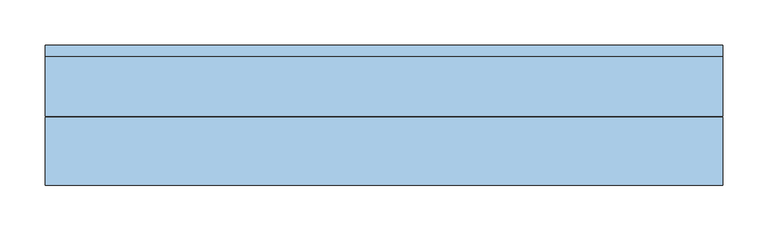
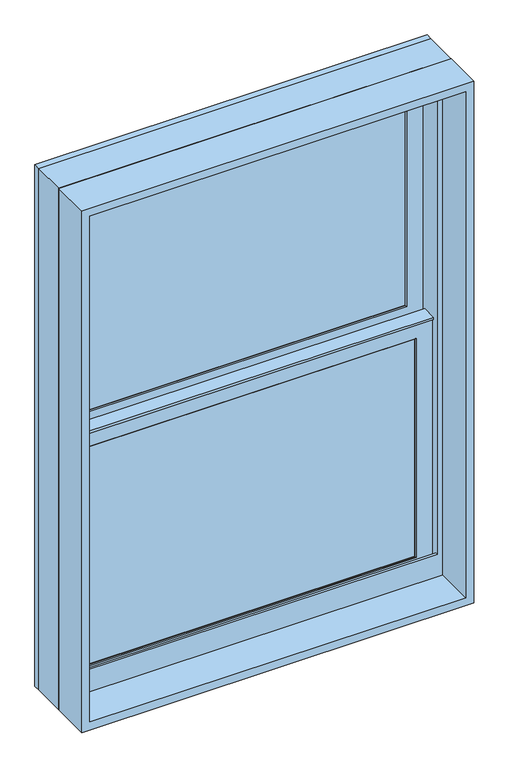
"""IFC4 building model written with IfcOpenShell, lengths in millimetres: window geometry, Window-Double_Hung-Marvin-Essential : ESDH2636."""

from ifc_helpers import new_model, si_unit, frame, origin, place, context, project, spatial, polyline, outline, extrude, faceted_brep, source, transform, mapped, element, save


def window_8203a103(model_context):
    return source(origin(), model_context, "Body", "SolidModel", [
        extrude(outline(polyline([(115.3583333, 20.6375), (115.3583333, 15.875), (96.3083333, 15.875), (96.3083333, 20.6375), (115.3583333, 20.6375)])), frame((0.0, 0.0, 1441.45), z_axis=(0.0, 0.0, 1.0), x_axis=(1.0, 0.0, 0.0)), (0.0, 0.0, 1.0), 450.85),
        extrude(outline(polyline([(-96.3083333, 20.6375), (-96.3083333, 15.875), (-115.3583333, 15.875), (-115.3583333, 20.6375), (-96.3083333, 20.6375)])), frame((0.0, 0.0, 1441.45), z_axis=(0.0, 0.0, 1.0), x_axis=(1.0, 0.0, 0.0)), (0.0, 0.0, 1.0), 450.85),
        extrude(outline(polyline([(317.5, 20.6375), (317.5, 15.875), (-317.5, 15.875), (-317.5, 20.6375), (317.5, 20.6375)])), frame((0.0, 0.0, 1657.35), z_axis=(0.0, 0.0, 1.0), x_axis=(1.0, 0.0, 0.0)), (0.0, 0.0, 1.0), 19.05),
        extrude(outline(polyline([(-115.3583333, 46.83125), (-115.3583333, 51.59375), (-96.3083333, 51.59375), (-96.3083333, 46.83125), (-115.3583333, 46.83125)])), frame((0.0, 0.0, 1930.4), z_axis=(0.0, 0.0, 1.0), x_axis=(1.0, 0.0, 0.0)), (0.0, 0.0, 1.0), 450.85),
        extrude(outline(polyline([(96.3083333, 46.83125), (96.3083333, 51.59375), (115.3583333, 51.59375), (115.3583333, 46.83125), (96.3083333, 46.83125)])), frame((0.0, 0.0, 1930.4), z_axis=(0.0, 0.0, 1.0), x_axis=(1.0, 0.0, 0.0)), (0.0, 0.0, 1.0), 450.85),
        extrude(outline(polyline([(-317.5, 46.83125), (-317.5, 51.59375), (317.5, 51.59375), (317.5, 46.83125), (-317.5, 46.83125)])), frame((0.0, 0.0, 2146.3), z_axis=(0.0, 0.0, 1.0), x_axis=(1.0, 0.0, 0.0)), (0.0, 0.0, 1.0), 19.05),
        extrude(outline(polyline([(115.3583333, 20.6375), (96.3083333, 20.6375), (96.3083333, 25.4), (115.3583333, 25.4), (115.3583333, 20.6375)])), frame((0.0, 0.0, 1441.45), z_axis=(0.0, 0.0, 1.0), x_axis=(1.0, 0.0, 0.0)), (0.0, 0.0, 1.0), 450.85),
        extrude(outline(polyline([(-96.3083333, 20.6375), (-115.3583333, 20.6375), (-115.3583333, 25.4), (-96.3083333, 25.4), (-96.3083333, 20.6375)])), frame((0.0, 0.0, 1441.45), z_axis=(0.0, 0.0, 1.0), x_axis=(1.0, 0.0, 0.0)), (0.0, 0.0, 1.0), 450.85),
        extrude(outline(polyline([(317.5, 20.6375), (-317.5, 20.6375), (-317.5, 25.4), (317.5, 25.4), (317.5, 20.6375)])), frame((0.0, 0.0, 1657.35), z_axis=(0.0, 0.0, 1.0), x_axis=(1.0, 0.0, 0.0)), (0.0, 0.0, 1.0), 19.05),
        extrude(outline(polyline([(-115.3583333, 56.35625), (-96.3083333, 56.35625), (-96.3083333, 51.59375), (-115.3583333, 51.59375), (-115.3583333, 56.35625)])), frame((0.0, 0.0, 1930.4), z_axis=(0.0, 0.0, 1.0), x_axis=(1.0, 0.0, 0.0)), (0.0, 0.0, 1.0), 450.85),
        extrude(outline(polyline([(96.3083333, 56.35625), (115.3583333, 56.35625), (115.3583333, 51.59375), (96.3083333, 51.59375), (96.3083333, 56.35625)])), frame((0.0, 0.0, 1930.4), z_axis=(0.0, 0.0, 1.0), x_axis=(1.0, 0.0, 0.0)), (0.0, 0.0, 1.0), 450.85),
        extrude(outline(polyline([(-317.5, 56.35625), (317.5, 56.35625), (317.5, 51.59375), (-317.5, 51.59375), (-317.5, 56.35625)])), frame((0.0, 0.0, 2146.3), z_axis=(0.0, 0.0, 1.0), x_axis=(1.0, 0.0, 0.0)), (0.0, 0.0, 1.0), 19.05),
        faceted_brep([(-344.4875, 5.6780605, 1922.3351748), (-344.4875, 5.6780605, 1917.7), (344.4875, 5.6780605, 1917.7), (344.4875, 5.6780605, 1922.3351748), (-344.4875, 34.8118605, 1922.3351748), (344.4875, 34.8118605, 1922.3351748), (344.4875, 34.8118605, 1917.7), (-344.4875, 34.8118605, 1917.7), (-344.4875, 30.1625, 1917.7), (-344.4875, 30.1625, 1414.4625), (-344.4875, 8.9241104, 1414.4625), (-344.4875, 8.9241104, 1917.7), (344.4875, 8.9241104, 1917.7), (344.4875, 30.1625, 1917.7), (344.4875, 8.9241104, 1414.4625), (344.4875, 30.1625, 1414.4625), (-328.6034752, 11.90625, 1903.4034752), (-328.6034752, 30.1625, 1903.4034752), (328.6034752, 30.1625, 1903.4034752), (328.6034752, 11.90625, 1903.4034752), (-311.94375, 10.4662439, 1886.74375), (-311.94375, 11.90625, 1886.74375), (311.94375, 11.90625, 1886.74375), (311.94375, 10.4662439, 1886.74375), (313.4858834, 8.9241104, 1888.2858834), (-313.4858834, 8.9241104, 1888.2858834), (328.6034752, 30.1625, 1430.3465248), (328.6034752, 11.90625, 1430.3465248), (311.94375, 11.90625, 1447.00625), (311.94375, 10.4662439, 1447.00625), (313.4858834, 8.9241104, 1445.4641166), (-328.6034752, 30.1625, 1430.3465248), (-328.6034752, 11.90625, 1430.3465248), (-311.94375, 11.90625, 1447.00625), (-311.94375, 10.4662439, 1447.00625), (-313.4858834, 8.9241104, 1445.4641166)], [[[0, 1, 2, 3]], [[4, 5, 6, 7]], [[1, 0, 4, 7, 8, 9, 10, 11]], [[2, 1, 11, 12]], [[7, 6, 13, 8]], [[3, 2, 12, 14, 15, 13, 6, 5]], [[0, 3, 5, 4]], [[16, 17, 18, 19]], [[20, 21, 22, 23]], [[20, 23, 24, 25]], [[19, 18, 26, 27]], [[23, 22, 28, 29]], [[24, 23, 29, 30]], [[27, 26, 31, 32]], [[29, 28, 33, 34]], [[30, 29, 34, 35]], [[15, 14, 10, 9]], [[15, 9, 8, 13], [18, 17, 31, 26]], [[17, 16, 32, 31]], [[16, 19, 27, 32], [22, 21, 33, 28]], [[21, 20, 34, 33]], [[20, 25, 35, 34]], [[10, 14, 12, 11], [25, 24, 30, 35]]]),
        extrude(outline(polyline([(38.5955581, 1903.4125), (33.5778968, 1903.4125), (33.5778968, 1905.0), (39.9405976, 1905.0), (39.9405976, 1903.4125), (61.515625, 1903.4125), (47.6307501, 1900.0975159), (38.5955581, 1900.0975159), (38.5955581, 1903.4125)])), frame((-344.4875, 0.0, 0.0), z_axis=(1.0, 0.0, 0.0), x_axis=(0.0, 1.0, 0.0)), (0.0, 0.0, 1.0), 688.975),
        faceted_brep([(374.65, 0.0, 1384.3), (374.65, 0.0, 2438.4), (-374.65, 0.0, 2438.4), (-374.65, 0.0, 1384.3), (348.45625, 0.0, 1445.41875), (-348.45625, 0.0, 1445.41875), (-348.45625, 0.0, 2412.20625), (348.45625, 0.0, 2412.20625), (348.45625, 3.96875, 1384.3), (-348.45625, 3.96875, 1384.3), (-348.45625, 3.96875, 1445.41875), (348.45625, 3.96875, 1445.41875), (-374.65, 65.6828125, 1384.3), (-348.45625, 65.6828125, 1384.3), (348.45625, 65.6828125, 1384.3), (374.65, 65.6828125, 1384.3), (-374.65, 65.6828125, 2438.4), (374.65, 65.6828125, 2438.4), (348.45625, 65.6828125, 2412.20625), (-348.45625, 65.6828125, 2412.20625)], [[[0, 1, 2, 3], [4, 5, 6, 7]], [[8, 9, 10, 11]], [[5, 4, 11, 10]], [[0, 3, 12, 13, 9, 8, 14, 15]], [[13, 12, 16, 17, 15, 14, 18, 19]], [[13, 19, 6, 5, 10, 9]], [[7, 6, 19, 18]], [[18, 14, 8, 11, 4, 7]], [[1, 0, 15, 17]], [[2, 1, 17, 16]], [[3, 2, 16, 12]]]),
        faceted_brep([(348.45625, 30.1625, 1911.35), (346.86875, 30.1625, 1911.35), (346.86875, 30.1625, 1408.6544613), (348.45625, 30.1625, 1408.6544613), (-346.86875, 30.1625, 1911.35), (-348.45625, 30.1625, 1911.35), (-348.45625, 30.1625, 1408.6544613), (-346.86875, 30.1625, 1408.6544613), (346.86875, 63.5, 1911.35), (348.45625, 63.5, 1911.35), (348.45625, 63.5, 1402.1743077), (346.86875, 63.5, 1402.1743077), (-348.45625, 63.5, 1911.35), (-346.86875, 63.5, 1911.35), (-346.86875, 63.5, 1402.1743077), (-348.45625, 63.5, 1402.1743077), (359.7108932, 3.96875, 1413.7460105), (359.7108932, 3.96875, 1384.3), (359.7108932, 65.6828125, 1384.3), (359.7108932, 65.6828125, 1401.750012), (-359.7108932, 3.96875, 1384.3), (-359.7108932, 3.96875, 1413.7460105), (-359.7108932, 65.6828125, 1401.750012), (-359.7108932, 65.6828125, 1384.3), (359.7108932, 78.58125, 1399.2428097), (-359.7108932, 78.58125, 1399.2428097), (-357.6971252, 68.2348864, 1401.2539391), (-339.73135, 68.2348864, 1401.2539391), (-339.73135, 65.6828125, 1401.750012), (339.73135, 65.6828125, 1401.750012), (339.73135, 68.2348864, 1401.2539391), (357.6971252, 68.2348864, 1401.2539391), (-374.65, 65.6828125, 1384.3), (-374.65, 78.5948249, 1384.3), (374.65, 78.5948249, 1384.3), (374.65, 65.6828125, 1384.3), (-374.65, 78.58125, 2438.4), (374.65, 78.58125, 2438.4), (359.7108932, 78.58125, 2423.4608932), (-359.7108932, 78.58125, 2423.4608932), (-374.65, 65.6828125, 2438.4), (-357.6971252, 68.2348864, 2421.4471252), (357.6971252, 68.2348864, 2421.4471252), (339.73135, 68.2348864, 2403.48135), (-339.73135, 68.2348864, 2403.48135), (-339.73135, 65.6828125, 2403.48135), (339.73135, 65.6828125, 2403.48135), (374.65, 65.6828125, 2438.4)], [[[0, 1, 2, 3]], [[4, 5, 6, 7]], [[8, 9, 10, 11]], [[12, 13, 14, 15]], [[1, 8, 11, 2]], [[9, 0, 3, 10]], [[1, 0, 9, 8]], [[5, 4, 13, 12]], [[5, 12, 15, 6]], [[13, 4, 7, 14]], [[16, 17, 18, 19]], [[20, 21, 22, 23]], [[24, 25, 26, 27, 28, 22, 21, 16, 19, 29, 30, 31], [3, 2, 11, 10], [7, 6, 15, 14]], [[17, 16, 21, 20]], [[17, 20, 23, 32, 33, 34, 35, 18]], [[34, 33, 36, 37], [25, 24, 38, 39]], [[33, 32, 40, 36]], [[39, 41, 26, 25]], [[41, 42, 31, 30, 43, 44, 27, 26]], [[44, 45, 28, 27]], [[40, 32, 23, 22, 28, 45, 46, 29, 19, 18, 35, 47]], [[36, 40, 47, 37]], [[39, 38, 42, 41]], [[44, 43, 46, 45]], [[34, 37, 47, 35]], [[42, 38, 24, 31]], [[46, 43, 30, 29]]]),
        extrude(outline(polyline([(324.64375, 11.90625), (-324.64375, 11.90625), (-324.64375, 15.08125), (324.64375, 15.08125), (324.64375, 11.90625)])), frame((0.0, 0.0, 1434.30625), z_axis=(0.0, 0.0, 1.0), x_axis=(1.0, 0.0, 0.0)), (0.0, 0.0, 1.0), 465.1375),
        extrude(outline(polyline([(324.64375, 42.8625), (-324.64375, 42.8625), (-324.64375, 46.0375), (324.64375, 46.0375), (324.64375, 42.8625)])), frame((0.0, 0.0, 1923.25625), z_axis=(0.0, 0.0, 1.0), x_axis=(1.0, 0.0, 0.0)), (0.0, 0.0, 1.0), 465.1375),
        faceted_brep([(-311.94375, 31.194477, 1886.74375), (-313.4858834, 32.7366104, 1888.2858834), (313.4858834, 32.7366104, 1888.2858834), (311.94375, 31.194477, 1886.74375), (-311.94375, 30.1625, 1886.74375), (311.94375, 30.1625, 1886.74375), (-344.4875, 32.7366104, 1919.2875), (-344.4875, 30.1625, 1919.2875), (344.4875, 30.1625, 1919.2875), (344.4875, 32.7366104, 1919.2875), (313.4858834, 32.7366104, 1445.4641166), (311.94375, 31.194477, 1447.00625), (311.94375, 30.1625, 1447.00625), (344.4875, 30.1625, 1414.4625), (344.4875, 32.7366104, 1414.4625), (-313.4858834, 32.7366104, 1445.4641166), (-311.94375, 31.194477, 1447.00625), (-311.94375, 30.1625, 1447.00625), (-344.4875, 30.1625, 1414.4625), (-344.4875, 32.7366104, 1414.4625)], [[[0, 1, 2, 3]], [[4, 0, 3, 5]], [[6, 7, 8, 9]], [[3, 2, 10, 11]], [[5, 3, 11, 12]], [[9, 8, 13, 14]], [[11, 10, 15, 16]], [[12, 11, 16, 17]], [[14, 13, 18, 19]], [[9, 14, 19, 6], [1, 15, 10, 2]], [[16, 15, 1, 0]], [[17, 16, 0, 4]], [[7, 18, 13, 8], [5, 12, 17, 4]], [[19, 18, 7, 6]]]),
        faceted_brep([(-328.6034752, 42.8625, 2392.3534752), (-328.6034752, 61.11875, 2392.3534752), (328.6034752, 61.11875, 2392.3534752), (328.6034752, 42.8625, 2392.3534752), (-311.94375, 41.4224939, 2375.69375), (-311.94375, 42.8625, 2375.69375), (311.94375, 42.8625, 2375.69375), (311.94375, 41.4224939, 2375.69375), (-313.4858834, 39.8803604, 2377.2358834), (313.4858834, 39.8803604, 2377.2358834), (-344.4875, 61.11875, 2408.2375), (-344.4875, 39.8803604, 2408.2375), (344.4875, 39.8803604, 2408.2375), (344.4875, 61.11875, 2408.2375), (328.6034752, 61.11875, 1919.2965248), (328.6034752, 42.8625, 1919.2965248), (311.94375, 42.8625, 1935.95625), (311.94375, 41.4224939, 1935.95625), (313.4858834, 39.8803604, 1934.4141166), (344.4875, 39.8803604, 1903.4125), (344.4875, 61.11875, 1903.4125), (-328.6034752, 61.11875, 1919.2965248), (-328.6034752, 42.8625, 1919.2965248), (-311.94375, 42.8625, 1935.95625), (-311.94375, 41.4224939, 1935.95625), (-313.4858834, 39.8803604, 1934.4141166), (-344.4875, 39.8803604, 1903.4125), (-344.4875, 61.11875, 1903.4125)], [[[0, 1, 2, 3]], [[4, 5, 6, 7]], [[8, 4, 7, 9]], [[10, 11, 12, 13]], [[3, 2, 14, 15]], [[7, 6, 16, 17]], [[9, 7, 17, 18]], [[13, 12, 19, 20]], [[15, 14, 21, 22]], [[17, 16, 23, 24]], [[18, 17, 24, 25]], [[20, 19, 26, 27]], [[13, 20, 27, 10], [1, 21, 14, 2]], [[22, 21, 1, 0]], [[3, 15, 22, 0], [5, 23, 16, 6]], [[24, 23, 5, 4]], [[25, 24, 4, 8]], [[11, 26, 19, 12], [9, 18, 25, 8]], [[27, 26, 11, 10]]]),
        faceted_brep([(-344.4875, 61.11875, 1903.4125), (-344.4875, 63.6928604, 1903.4125), (344.4875, 63.6928604, 1903.4125), (344.4875, 61.11875, 1903.4125), (-311.94375, 62.150727, 1935.95625), (-311.94375, 61.11875, 1935.95625), (311.94375, 61.11875, 1935.95625), (311.94375, 62.150727, 1935.95625), (-313.4858834, 63.6928604, 1934.4141166), (313.4858834, 63.6928604, 1934.4141166), (344.4875, 63.6928604, 2408.2375), (344.4875, 61.11875, 2408.2375), (311.94375, 61.11875, 2375.69375), (311.94375, 62.150727, 2375.69375), (313.4858834, 63.6928604, 2377.2358834), (-344.4875, 63.6928604, 2408.2375), (-344.4875, 61.11875, 2408.2375), (-311.94375, 61.11875, 2375.69375), (-311.94375, 62.150727, 2375.69375), (-313.4858834, 63.6928604, 2377.2358834)], [[[0, 1, 2, 3]], [[4, 5, 6, 7]], [[8, 4, 7, 9]], [[3, 2, 10, 11]], [[7, 6, 12, 13]], [[9, 7, 13, 14]], [[11, 10, 15, 16]], [[13, 12, 17, 18]], [[14, 13, 18, 19]], [[16, 15, 1, 0]], [[3, 11, 16, 0], [5, 17, 12, 6]], [[18, 17, 5, 4]], [[19, 18, 4, 8]], [[1, 15, 10, 2], [9, 14, 19, 8]]]),
        extrude(outline(polyline([(324.64375, 26.19375), (-324.64375, 26.19375), (-324.64375, 30.1625), (324.64375, 30.1625), (324.64375, 26.19375)])), frame((0.0, 0.0, 1434.30625), z_axis=(0.0, 0.0, 1.0), x_axis=(1.0, 0.0, 0.0)), (0.0, 0.0, 1.0), 465.1375),
        extrude(outline(polyline([(324.64375, 57.15), (-324.64375, 57.15), (-324.64375, 61.11875), (324.64375, 61.11875), (324.64375, 57.15)])), frame((0.0, 0.0, 1923.25625), z_axis=(0.0, 0.0, 1.0), x_axis=(1.0, 0.0, 0.0)), (0.0, 0.0, 1.0), 465.1375),
        extrude(outline(polyline([(2438.4, 374.65), (2438.4, -374.65), (1384.3, -374.65), (1384.3, 374.65), (2438.4, 374.65)]), holes=[polyline([(2422.525, 358.775), (1400.175, 358.775), (1400.175, -358.775), (2422.525, -358.775), (2422.525, 358.775)])]), frame((0.0, -76.2, 0.0), z_axis=(0.0, 1.0, 0.0), x_axis=(0.0, 0.0, 1.0)), (0.0, 0.0, 1.0), 75.40625),
    ])


if __name__ == "__main__":
    model = new_model("IFC4")
    model_context = context("Model", 3, world=origin())
    ifc_project = project(units=[si_unit("LENGTHUNIT", "METRE", prefix="MILLI")], contexts=[model_context])
    site = spatial("IfcSite", under=ifc_project)
    building = spatial("IfcBuilding", under=site)
    placement = place(None, origin())
    window_shape = window_8203a103(model_context)
    element("IfcWindow", 1, ObjectType="Window-Double_Hung-Marvin-Essential : ESDH2636", at=placement, inside=building, context=model_context, shape_type="MappedRepresentation", body=[
        mapped(window_shape, transform((0.0, 0.0, 0.0), x_axis=(1.0, 0.0, 0.0), y_axis=(0.0, 1.0, 0.0), z_axis=(0.0, 0.0, 1.0))),
    ])
    save(model, "model.ifc")

# Revit data of these elements
# Type "Window-Double_Hung-Marvin-Essential : ESDH2636"
#   Type Mark = "42"
#   Window Type = "Essential Double Hung"
#   Product data url = "https://bimobject.com/marvin-windows-and-doors/product/marvin-dhwau"
#   Product Guid = "c4a96547-874c-4385-91dc-a058adc19d98"
#   Frame = "All Ultrex"
#   Egress Window = "No"
#   URL = "www.marvin.com"
#   Model = "ESDH2636"
#   Manufacturer = "Marvin Windows and Doors"
#   Label Egress = ""
#   Glass Type = "IG Low E II with Argon"
#   Design Pressure = "DP50"
#   Description = "3042 DBHG"
#   Analytic Construction = "<None>"
#   Prairie Corner Width = 0' - 4"
#   Prairie Corner Height = 0' - 4"
#   Egress Width = 2' - 2 9/16"
#   Egress Height = 1' - 4 27/128"
#   Rough Width = 2' - 6"
#   Rough Height = 3' - 6"
#   Nominal Width = 2' - 6"
#   Nominal Height = 3' - 6"
#   Inset to Installation Flange [instance default] = 0' - 1"
#   Height = 3' - 5 1/2"
#   Egress Area = 2.9903 SF
#   Default Head Height = 8' - 0"
#   Width = 2' - 5 1/2"
#   Daylight Area = 5.90609 SF
#   DLO Width = 2' - 0 9/16"
#   DLO Height = 1' - 5 5/16"
#   Muntins Top Sash = yes
#   Lites Wide Top Sash = 3
#   Lites Wide Bottom Sash = 3
#   Lites High Top Sash = 2
#   Lites High Bottom Sash = 2
#   Lite Cut Prairie 9 = no
#   Lite Cut HV Grid = yes
#   Muntins Bottom Sash = yes
#   Label Visibility = no
#   Jamb Extension Visibility = yes
#   Edition number = 1
#   Interior Material = Ultrex-Marvin-Stonewhite
#   Glazing Material = Glass-Marvin-IG Low E II with Argon
#   Cladding Material = Ultrex-Marvin-Pebblegray
#   Wall Closure = (empty or 0)
#   Assembly Code = ""
# Element 1 (IfcWindow, "Window-Double_Hung-Marvin-Essential : ESDH2636")
#   Materials on its faces: "Ultrex-Marvin-Pebblegray", "Ultrex-Marvin-Stonewhite", "Glass-Marvin-IG Low E II with Argon"
# Materials
#   "Ultrex-Marvin-Stonewhite": class "Paint", colour RGB 250 251 245, transparency 0
#   "Glass-Marvin-IG Low E II with Argon": class "Glass", colour RGB 0 128 192, transparency 0.85
#   "Ultrex-Marvin-Pebblegray": class "Paint", colour RGB 189 185 173, transparency 0
